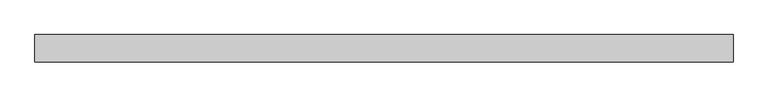
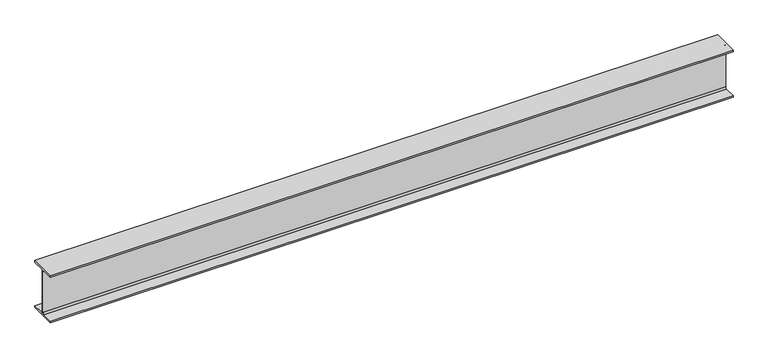
"""IFC4 building model written with IfcOpenShell, lengths in millimetres: beam geometry, Old_Steel Beam_H-KSD3502 : H_SB_ASB_H-200×200x8x12."""

from ifc_helpers import new_model, si_unit, point, frame, frame_2d, origin, place, context, project, spatial, polyline, circle_curve, trimmed, segment, composite_curve, outline, extrude, source, transform, mapped, element, save


def beam_7a6e46e6(model_context):
    return source(origin(), model_context, "Body", "SweptSolid", [
        extrude(outline(composite_curve([segment(polyline([(82.5, -141.5), (82.5, -151.7), (-82.5, -151.7), (-82.5, -141.5), (-11.9, -141.5)]), True, "CONTINUOUS"), segment(trimmed(circle_curve(frame_2d((-11.9, -132.6)), 8.9), [point((-11.9, -141.5))], [point((-3.0, -132.6))], True, "CARTESIAN"), True, "CONTINUOUS"), segment(polyline([(-3.0, -132.6), (-3.0, 132.6)]), True, "CONTINUOUS"), segment(trimmed(circle_curve(frame_2d((-11.9, 132.6)), 8.9), [point((-3.0, 132.6))], [point((-11.9, 141.5))], True, "CARTESIAN"), True, "CONTINUOUS"), segment(polyline([(-11.9, 141.5), (-82.5, 141.5), (-82.5, 151.7), (82.5, 151.7), (82.5, 141.5), (11.9, 141.5)]), True, "CONTINUOUS"), segment(trimmed(circle_curve(frame_2d((11.9, 132.6)), 8.9), [point((11.9, 141.5))], [point((3.0, 132.6))], True, "CARTESIAN"), True, "CONTINUOUS"), segment(polyline([(3.0, 132.6), (3.0, -132.6)]), True, "CONTINUOUS"), segment(trimmed(circle_curve(frame_2d((11.9, -132.6)), 8.9), [point((3.0, -132.6))], [point((11.9, -141.5))], True, "CARTESIAN"), True, "CONTINUOUS"), segment(polyline([(11.9, -141.5), (82.5, -141.5)]), True, "CONTINUOUS")], self_intersect=False)), frame((-2019.0792916, 0.0, 0.0), z_axis=(1.0, 0.0, 0.0), x_axis=(0.0, 1.0, 0.0)), (0.0, 0.0, 1.0), 4179.9604005),
    ])


if __name__ == "__main__":
    model = new_model("IFC4")
    model_context = context("Model", 3, world=origin())
    ifc_project = project(units=[si_unit("LENGTHUNIT", "METRE", prefix="MILLI")], contexts=[model_context])
    site = spatial("IfcSite", under=ifc_project)
    building = spatial("IfcBuilding", under=site)
    placement = place(None, origin())
    beam_shape = beam_7a6e46e6(model_context)
    element("IfcBeam", 1, ObjectType="Old_Steel Beam_H-KSD3502 : H_SB_ASB_H-200×200x8x12", at=placement, inside=building, context=model_context, shape_type="MappedRepresentation", body=[
        mapped(beam_shape, transform((0.0, 0.0, 0.0), x_axis=(1.0, 0.0, 0.0), y_axis=(0.0, 1.0, 0.0), z_axis=(0.0, 0.0, 1.0))),
    ])
    save(model, "model.ifc")

# Revit data of these elements
# Type "Old_Steel Beam_H-KSD3502 : H_SB_ASB_H-200×200x8x12"
#   Width = 20.0 cm
#   Web Thickness = 0.8 cm
#   Web Fillet = 1.3 cm
#   Warping Constant = 141376.0 cm⁶
#   Torsional Moment of Inertia = 26.2485 cm⁴
#   Torsional Modulus = 1.0 cm³
#   Section Area = 63.53 cm²
#   Plastic Modulus weak axis = 244.0 cm³
#   Plastic Modulus strong axis = 525.0 cm³
#   Perimeter = 1.16 m²/m
#   Nominal Weight = 49.90 kgf/m
#   Moment of Inertia weak axis = 1600.00 cm⁴
#   Moment of Inertia strong axis = 4720.00 cm⁴
#   Height = 20.0 cm
#   Flange Thickness = 1.2 cm
#   Elastic Modulus weak axis = 160.0 cm³
#   Elastic Modulus strong axis = 472.0 cm³
#   Centroid Vertical = 10.0 cm
#   Centroid Horizontal = 10.0 cm
#   Length [instance default] = 1.5240 m
#   Structural Material [instance default] = Steel, 45-345
#   Assembly Code = ""
# Element 1 (IfcBeam, "Old_Steel Beam_H-KSD3502 : H_SB_ASB_H-200×200x8x12")
#   Structural Material = none
# Materials
#   "Steel, 45-345": class "Metal", colour RGB 189 187 185, transparency 0, Description = "Steel 345 MPa", Cost = 0
